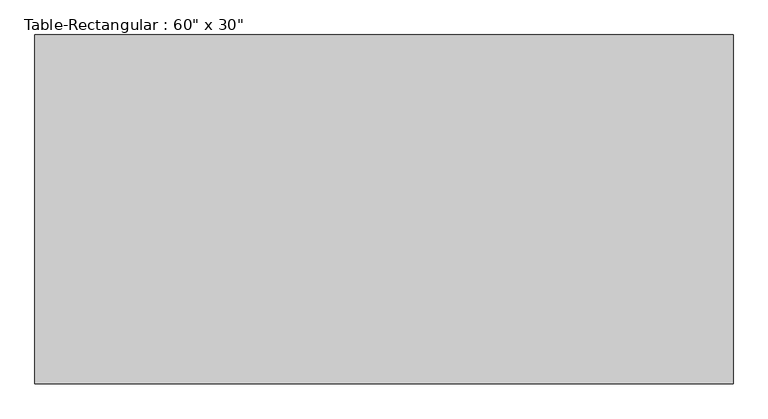
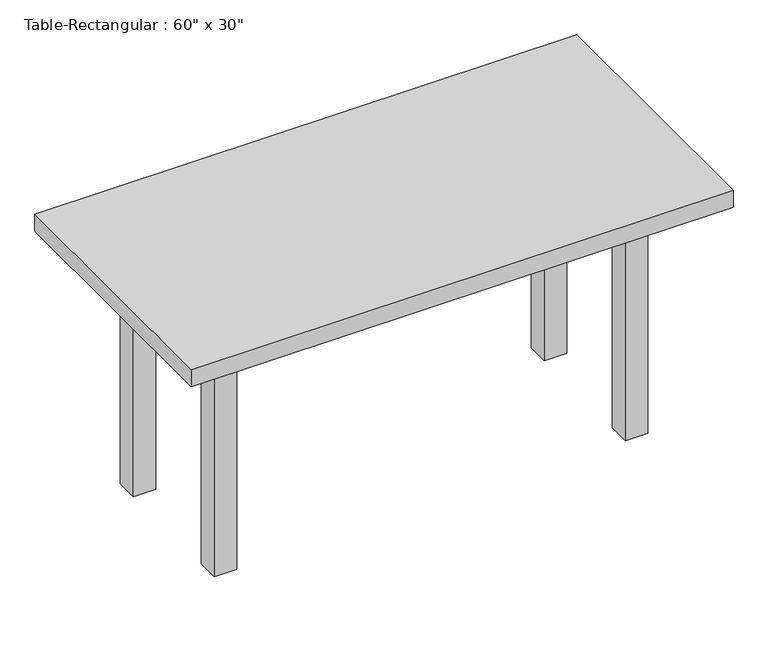
"""IFC4 building model written with IfcOpenShell, lengths in millimetres: furniture geometry."""

from ifc_helpers import new_model, si_unit, frame, origin, origin_with_axes, place, context, project, spatial, polyline, outline, extrude, source, transform, mapped, element, save


def furniture_d900495b(model_context):
    return source(origin(), model_context, "Body", "SweptSolid", [
        extrude(outline(polyline([(546.1, 190.5), (546.1, 165.1), (-546.1, 165.1), (-546.1, 190.5), (546.1, 190.5)])), frame((0.0, 0.0, 609.6), z_axis=(0.0, 0.0, 1.0), x_axis=(1.0, 0.0, 0.0)), (0.0, 0.0, 1.0), 101.6),
        extrude(outline(polyline([(546.1, -190.5), (-546.1, -190.5), (-546.1, -165.1), (546.1, -165.1), (546.1, -190.5)])), frame((0.0, 0.0, 609.6), z_axis=(0.0, 0.0, 1.0), x_axis=(1.0, 0.0, 0.0)), (0.0, 0.0, 1.0), 101.6),
        extrude(outline(polyline([(-558.8, -165.1), (-584.2, -165.1), (-584.2, 165.1), (-558.8, 165.1), (-558.8, -165.1)])), frame((0.0, 0.0, 609.6), z_axis=(0.0, 0.0, 1.0), x_axis=(1.0, 0.0, 0.0)), (0.0, 0.0, 1.0), 101.6),
        extrude(outline(polyline([(558.8, -165.1), (558.8, 165.1), (584.2, 165.1), (584.2, -165.1), (558.8, -165.1)])), frame((0.0, 0.0, 609.6), z_axis=(0.0, 0.0, 1.0), x_axis=(1.0, 0.0, 0.0)), (0.0, 0.0, 1.0), 101.6),
        extrude(outline(polyline([(762.0, 381.0), (762.0, -381.0), (-762.0, -381.0), (-762.0, 381.0), (762.0, 381.0)])), frame((0.0, 0.0, 711.2), z_axis=(0.0, 0.0, 1.0), x_axis=(1.0, 0.0, 0.0)), (0.0, 0.0, 1.0), 50.8),
        extrude(outline(polyline([(-546.1, 228.6), (-546.1, 165.1), (-609.6, 165.1), (-609.6, 228.6), (-546.1, 228.6)])), origin_with_axes(), (0.0, 0.0, 1.0), 711.2),
        extrude(outline(polyline([(546.1, 228.6), (609.6, 228.6), (609.6, 165.1), (546.1, 165.1), (546.1, 228.6)])), origin_with_axes(), (0.0, 0.0, 1.0), 711.2),
        extrude(outline(polyline([(-546.1, -228.6), (-609.6, -228.6), (-609.6, -165.1), (-546.1, -165.1), (-546.1, -228.6)])), origin_with_axes(), (0.0, 0.0, 1.0), 711.2),
        extrude(outline(polyline([(546.1, -228.6), (546.1, -165.1), (609.6, -165.1), (609.6, -228.6), (546.1, -228.6)])), origin_with_axes(), (0.0, 0.0, 1.0), 711.2),
    ])


if __name__ == "__main__":
    model = new_model("IFC4")
    model_context = context("Model", 3, world=origin())
    ifc_project = project(units=[si_unit("LENGTHUNIT", "METRE", prefix="MILLI")], contexts=[model_context])
    site = spatial("IfcSite", under=ifc_project)
    building = spatial("IfcBuilding", under=site)
    placement = place(None, origin())
    furniture_shape = furniture_d900495b(model_context)
    element("IfcFurniture", 1, ObjectType="Table-Rectangular : 60\" x 30\"", at=placement, inside=building, context=model_context, shape_type="MappedRepresentation", body=[
        mapped(furniture_shape, transform((0.0, 0.0, 0.0), x_axis=(1.0, 0.0, 0.0), y_axis=(0.0, 1.0, 0.0), z_axis=(0.0, 0.0, 1.0))),
    ])
    save(model, "model.ifc")

# Revit data of these elements
# Type "Table-Rectangular : 60\" x 30\""
#   Assembly Code = "E2020200"
#   Height = 2' - 6"
#   Length = 5' - 0"
#   Width = 2' - 6"
#   Base Material = Birch
#   Top Material = Birch
#   Default Elevation = 0
# Element 1 (IfcFurniture, "Table-Rectangular : 60\" x 30\"")
#   Materials on its faces: "Birch"
# Materials
#   "Birch": class "Wood", colour RGB 224 178 126, transparency 0, Description = "Betula Alleghaniensis", Cost = 0
